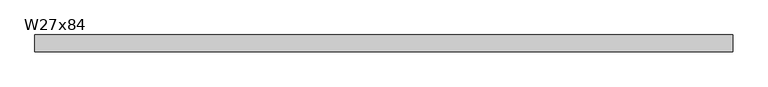
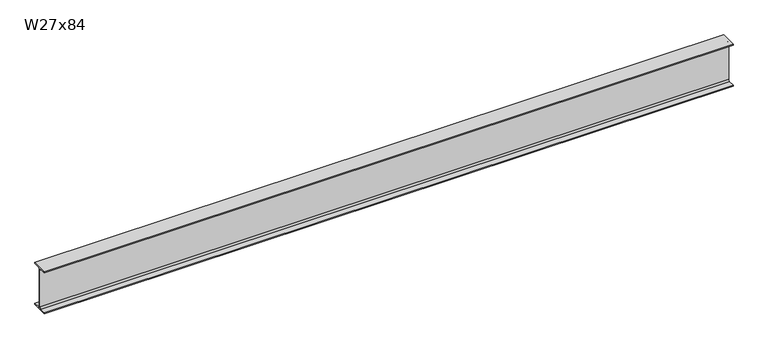
"""IFC4 building model written with IfcOpenShell, lengths in millimetres: beam geometry, RME W-Wide Flange : W27x84."""

from ifc_helpers import new_model, si_unit, point, frame, frame_2d, origin, place, context, project, spatial, polyline, circle_curve, trimmed, segment, composite_curve, outline, extrude, source, transform, mapped, element, save


def w27x84_458d2ca8(model_context):
    return source(origin(), model_context, "Body", "SweptSolid", [
        extrude(outline(composite_curve([segment(polyline([(127.0, -322.834), (127.0, -339.09), (-127.0, -339.09), (-127.0, -322.834), (-29.2735, -322.834)]), True, "CONTINUOUS"), segment(trimmed(circle_curve(frame_2d((-29.2735, -299.4025)), 23.4315), [point((-29.2735, -322.834))], [point((-5.842, -299.4025))], True, "CARTESIAN"), True, "CONTINUOUS"), segment(polyline([(-5.842, -299.4025), (-5.842, 299.4025)]), True, "CONTINUOUS"), segment(trimmed(circle_curve(frame_2d((-29.2735, 299.4025)), 23.4315), [point((-5.842, 299.4025))], [point((-29.2735, 322.834))], True, "CARTESIAN"), True, "CONTINUOUS"), segment(polyline([(-29.2735, 322.834), (-127.0, 322.834), (-127.0, 339.09), (127.0, 339.09), (127.0, 322.834), (29.2735, 322.834)]), True, "CONTINUOUS"), segment(trimmed(circle_curve(frame_2d((29.2735, 299.4025)), 23.4315), [point((29.2735, 322.834))], [point((5.842, 299.4025))], True, "CARTESIAN"), True, "CONTINUOUS"), segment(polyline([(5.842, 299.4025), (5.842, -299.4025)]), True, "CONTINUOUS"), segment(trimmed(circle_curve(frame_2d((29.2735, -299.4025)), 23.4315), [point((5.842, -299.4025))], [point((29.2735, -322.834))], True, "CARTESIAN"), True, "CONTINUOUS"), segment(polyline([(29.2735, -322.834), (127.0, -322.834)]), True, "CONTINUOUS")], self_intersect=False)), frame((-5223.7472842, 0.0, 0.0), z_axis=(1.0, 0.0, 0.0), x_axis=(0.0, 1.0, 0.0)), (0.0, 0.0, 1.0), 10561.7945684),
    ])


if __name__ == "__main__":
    model = new_model("IFC4")
    model_context = context("Model", 3, world=origin())
    ifc_project = project(units=[si_unit("LENGTHUNIT", "METRE", prefix="MILLI")], contexts=[model_context])
    site = spatial("IfcSite", under=ifc_project)
    building = spatial("IfcBuilding", under=site)
    placement = place(None, origin())
    w27x84_shape = w27x84_458d2ca8(model_context)
    element("IfcBeam", 1, ObjectType="RME W-Wide Flange : W27x84", at=placement, inside=building, context=model_context, shape_type="MappedRepresentation", body=[
        mapped(w27x84_shape, transform((0.0, 0.0, 0.0), x_axis=(1.0, 0.0, 0.0), y_axis=(0.0, 1.0, 0.0), z_axis=(0.0, 0.0, 1.0))),
    ])
    save(model, "model.ifc")

# Revit data of these elements
# Type "RME W-Wide Flange : W27x84"
#   WELD P [instance default] = ""
#   WELD LE [instance default] = ""
#   WELD D [instance default] = ""
#   TOP SECTION SIZE [instance default] = ""
#   TOP SECTION LENGTH [instance default] = ""
#   REMARKS [instance default] = ""
#   REINF TYPE [instance default] = ""
#   Nominal Size = "W24"
#   End Bearing Capacity [instance default] = ""
#   BOT SECTION SIZE [instance default] = ""
#   BOT SECTION LENGTH [instance default] = ""
#   Assembly Code = "B10"
#   W = 84
#   Start Extension Calculation [instance default] = 10' - 0"
#   Start Extension [instance default] = -0' - 0 1/2"
#   End Extension Calculation [instance default] = 10' - 0"
#   End Extension [instance default] = -0' - 0 1/2"
#   Length [instance default] = 5' - 0"
#   bf = 0' - 10"
#   d = 2' - 2.7"
#   k = 0' - 1 9/16"
#   k2 = 0' - 0.9225"
#   tf = 0' - 0.64"
#   tw = 0' - 0.46"
#   A = 0.172222 SF
#   Structural Material [instance default] = Metal - Steel - ASTM A992
# Element 1 (IfcBeam, "RME W-Wide Flange : W27x84")
#   Length = 35' - 0.31868"
#   Materials on its faces: "Metal - Steel - ASTM A992"
# Materials
#   "Metal - Steel - ASTM A992": class "Metal", colour RGB 255 128 0, transparency 0
